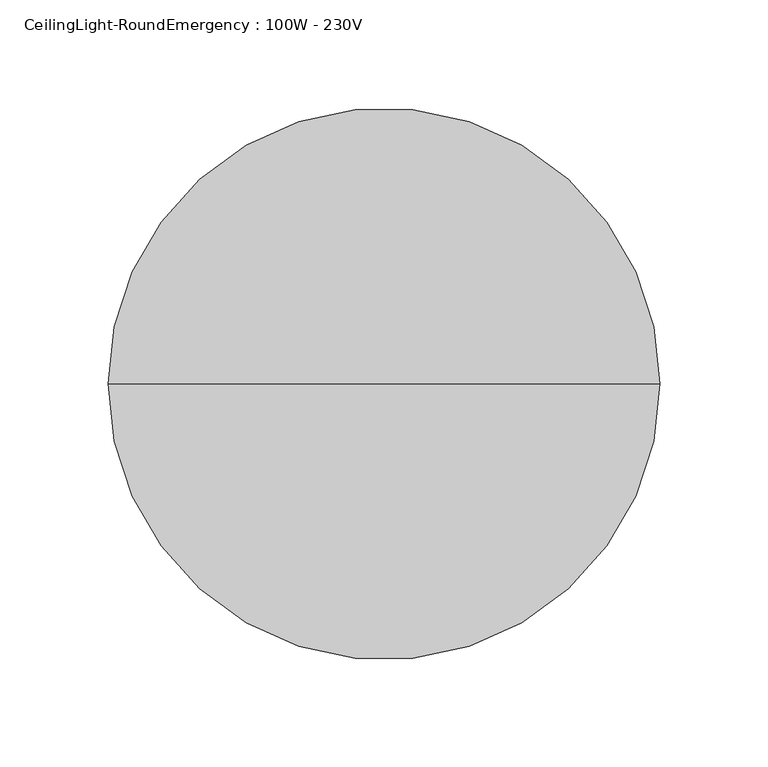
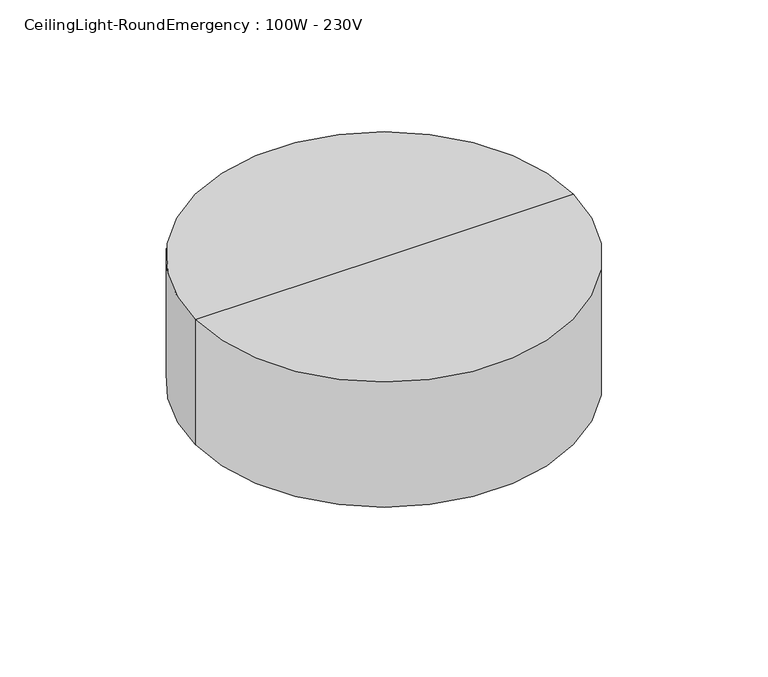
"""IFC4 building model written with IfcOpenShell, lengths in millimetres: light fixture geometry, CeilingLight-RoundEmergency : 100W - 230V."""

from ifc_helpers import new_model, si_unit, point, frame, origin, origin_2d, place, context, project, spatial, polyline, circle_curve, trimmed, segment, composite_curve, outline, extrude, source, transform, mapped, element, save
from ifc_brep_helpers import plane_surface, cylinder_surface, revolved_surface, advanced_brep


def ceilinglight_roundemergency_100w_230v_36b39b3f(model_context):
    return source(origin(), model_context, "Body", "SolidModel", [
        extrude(outline(composite_curve([segment(trimmed(circle_curve(origin_2d(), 82.55), [point((-82.55, 0.0))], [point((82.55, 0.0))], False, "CARTESIAN"), True, "CONTINUOUS"), segment(trimmed(circle_curve(origin_2d(), 82.55), [point((82.55, 0.0))], [point((-82.55, 0.0))], False, "CARTESIAN"), True, "CONTINUOUS")], self_intersect=False), holes=[composite_curve([segment(trimmed(circle_curve(origin_2d(), 76.2), [point((-76.2, 0.0))], [point((76.2, 0.0))], True, "CARTESIAN"), True, "CONTINUOUS"), segment(trimmed(circle_curve(origin_2d(), 76.2), [point((76.2, 0.0))], [point((-76.2, 0.0))], True, "CARTESIAN"), True, "CONTINUOUS")], self_intersect=False)]), frame((0.0, 0.0, -101.810254), z_axis=(0.0, 0.0, 1.0), x_axis=(1.0, 0.0, 0.0)), (0.0, 0.0, 1.0), 25.0),
        advanced_brep(
        [(127.0, 0.0, -74.6), (-127.0, 0.0, -74.6), (-127.0, 0.0, 14.3), (127.0, 0.0, 14.3), (76.2, 0.0, -74.6), (-76.2, 0.0, -74.6), (76.2, 0.0, -100.0), (-76.2, 0.0, -100.0), (73.025, 0.0, -100.0), (-73.025, 0.0, -100.0), (73.025, 0.0, -71.425), (-73.025, 0.0, -71.425), (123.825, 0.0, -71.425), (-123.825, 0.0, -71.425), (123.825, 0.0, 11.125), (-123.825, 0.0, 11.125), (0.0, 0.0, 11.125), (0.0, 0.0, 14.3)],
        [
            (0, 1, circle_curve(frame((0.0, 0.0, -74.6), z_axis=(0.0, 0.0, 1.0), x_axis=(-1.0, 0.0, 0.0)), 127.0)),
            (1, 2),
            (2, 3, circle_curve(frame((0.0, 0.0, 14.3), z_axis=(0.0, 0.0, -1.0), x_axis=(-1.0, 0.0, 0.0)), 127.0)),
            (3, 0),
            (1, 0, circle_curve(frame((0.0, 0.0, -74.6), z_axis=(0.0, 0.0, 1.0), x_axis=(-1.0, 0.0, 0.0)), 127.0)),
            (3, 2, circle_curve(frame((0.0, 0.0, 14.3), z_axis=(0.0, 0.0, -1.0), x_axis=(-1.0, 0.0, 0.0)), 127.0)),
            (4, 5, circle_curve(frame((0.0, 0.0, -74.6), z_axis=(0.0, 0.0, 1.0), x_axis=(-1.0, 0.0, 0.0)), 76.2)),
            (5, 1),
            (0, 4),
            (5, 4, circle_curve(frame((0.0, 0.0, -74.6), z_axis=(0.0, 0.0, 1.0), x_axis=(-1.0, 0.0, 0.0)), 76.2)),
            (6, 7, circle_curve(frame((0.0, 0.0, -100.0), z_axis=(0.0, 0.0, 1.0), x_axis=(-1.0, 0.0, 0.0)), 76.2)),
            (7, 5),
            (4, 6),
            (7, 6, circle_curve(frame((0.0, 0.0, -100.0), z_axis=(0.0, 0.0, 1.0), x_axis=(-1.0, 0.0, 0.0)), 76.2)),
            (8, 9, circle_curve(frame((0.0, 0.0, -100.0), z_axis=(0.0, 0.0, 1.0), x_axis=(-1.0, 0.0, 0.0)), 73.025)),
            (9, 7),
            (6, 8),
            (9, 8, circle_curve(frame((0.0, 0.0, -100.0), z_axis=(0.0, 0.0, 1.0), x_axis=(-1.0, 0.0, 0.0)), 73.025)),
            (10, 11, circle_curve(frame((0.0, 0.0, -71.425), z_axis=(0.0, 0.0, 1.0), x_axis=(-1.0, 0.0, 0.0)), 73.025)),
            (11, 9),
            (8, 10),
            (11, 10, circle_curve(frame((0.0, 0.0, -71.425), z_axis=(0.0, 0.0, 1.0), x_axis=(-1.0, 0.0, 0.0)), 73.025)),
            (12, 13, circle_curve(frame((0.0, 0.0, -71.425), z_axis=(0.0, 0.0, 1.0), x_axis=(-1.0, 0.0, 0.0)), 123.825)),
            (13, 11),
            (10, 12),
            (13, 12, circle_curve(frame((0.0, 0.0, -71.425), z_axis=(0.0, 0.0, 1.0), x_axis=(-1.0, 0.0, 0.0)), 123.825)),
            (14, 15, circle_curve(frame((0.0, 0.0, 11.125), z_axis=(0.0, 0.0, 1.0), x_axis=(-1.0, 0.0, 0.0)), 123.825)),
            (15, 13),
            (12, 14),
            (15, 14, circle_curve(frame((0.0, 0.0, 11.125), z_axis=(0.0, 0.0, 1.0), x_axis=(-1.0, 0.0, 0.0)), 123.825)),
            (16, 15),
            (14, 16),
            (2, 17),
            (17, 3),
        ],
        [
            cylinder_surface(frame((0.0, 0.0, 11.125), z_axis=(0.0, 0.0, -1.0), x_axis=(-1.0, 0.0, 0.0)), 127.0),
            plane_surface(frame((0.0, 0.0, -74.6), z_axis=(0.0, 0.0, -1.0), x_axis=(-1.0, 0.0, 0.0))),
            cylinder_surface(frame((0.0, 0.0, 11.125), z_axis=(0.0, 0.0, -1.0), x_axis=(-1.0, 0.0, 0.0)), 76.2),
            plane_surface(frame((0.0, 0.0, -100.0), z_axis=(0.0, 0.0, -1.0), x_axis=(-1.0, 0.0, 0.0))),
            revolved_surface(polyline([(-73.025, 0.0, -100.0), (-73.025, 0.0, -71.425)]), (0.0, 0.0, 11.125), (0.0, 0.0, -1.0)),
            plane_surface(frame((0.0, 0.0, -71.425), z_axis=(0.0, 0.0, 1.0), x_axis=(-1.0, 0.0, 0.0))),
            revolved_surface(polyline([(-123.825, 0.0, -71.425), (-123.825, 0.0, 11.125)]), (0.0, 0.0, 11.125), (0.0, 0.0, -1.0)),
            plane_surface(frame((0.0, 0.0, 11.125), z_axis=(0.0, 0.0, -1.0), x_axis=(-1.0, 0.0, 0.0))),
            plane_surface(frame((0.0, 0.0, 14.3), z_axis=(0.0, 0.0, 1.0), x_axis=(-1.0, 0.0, 0.0))),
        ],
        [
            (0, [[1, 2, 3, 4]]),
            (0, [[5, -4, 6, -2]]),
            (1, [[7, 8, -1, 9]]),
            (1, [[10, -9, -5, -8]]),
            (2, [[11, 12, -7, 13]]),
            (2, [[14, -13, -10, -12]]),
            (3, [[15, 16, -11, 17]]),
            (3, [[18, -17, -14, -16]]),
            (4, [[19, 20, -15, 21]]),
            (4, [[22, -21, -18, -20]]),
            (5, [[23, 24, -19, 25]]),
            (5, [[26, -25, -22, -24]]),
            (6, [[27, 28, -23, 29]]),
            (6, [[30, -29, -26, -28]]),
            (7, [[31, -27, 32]]),
            (7, [[-32, -30, -31]]),
            (8, [[-3, 33, 34]]),
            (8, [[-6, -34, -33]]),
        ],
    ),
    ])


if __name__ == "__main__":
    model = new_model("IFC4")
    model_context = context("Model", 3, world=origin())
    ifc_project = project(units=[si_unit("LENGTHUNIT", "METRE", prefix="MILLI")], contexts=[model_context])
    site = spatial("IfcSite", under=ifc_project)
    building = spatial("IfcBuilding", under=site)
    placement = place(None, origin())
    ceilinglight_roundemergency_100w_230v_shape = ceilinglight_roundemergency_100w_230v_36b39b3f(model_context)
    element("IfcLightFixture", 1, ObjectType="CeilingLight-RoundEmergency : 100W - 230V", at=placement, inside=building, context=model_context, shape_type="MappedRepresentation", body=[
        mapped(ceilinglight_roundemergency_100w_230v_shape, transform((0.0, 0.0, 0.0), x_axis=(1.0, 0.0, 0.0), y_axis=(0.0, 1.0, 0.0), z_axis=(0.0, 0.0, 1.0))),
    ])
    save(model, "model.ifc")

# Revit data of these elements
# Type "CeilingLight-RoundEmergency : 100W - 230V"
#   Type Mark = "CeilingLight-RoundEmergencyB"
#   Classification.OmniClass.21.Number = "21-04 50 40 50"
#   Classification.OmniClass.21.Description = "Lighting Fixtures"
#   Classification.UniFormat.II.Description = "Lighting Fixtures"
#   Classification.OmniClass.23.Number = "23-35 47 13"
#   Classification.OmniClass.23.Description = "Emergency Lighting"
#   Classification.UniFormat.II.Number = "D5040.50"
#   COBie.Type.CreatedBy = "info@mma.ie"
#   COBie.Type.CreatedOn = "2017-07-25T10:15:16"
#   COBie.Type.Name = "CeilingLight-RoundEmergencyB"
#   COBie.Type.Category = "23-35 47 13 : Emergency Lighting"
#   COBie.Type.Description = "CeilingLight-RoundEmergency_100W - 230V"
#   COBie.Type.AssetType = "Fixed"
#   COBie.Type.Manufacturer = ""
#   COBie.Type.ModelNumber = ""
#   Keynote = "26 52 00.B"
#   Lamp = "A-19"
#   Photometric Web File = "CLFR1A21.ies"
#   Assembly Code = "D5020220"
#   COBie.Type.ReplacementCost = 0
#   Wattage = 100 W
#   built-in parameter 1150110 = 1 (stored number, unit not read)
#   built-in parameter 1150109 = 1 (stored number, unit not read)
#   built-in parameter 1150113 = 1 (stored number, unit not read)
#   Tilt Angle = -90.00°
#   built-in parameter 1150115 = 1 (stored number, unit not read)
#   built-in parameter 1150105 = 139.261 (stored number, unit not read)
#   built-in parameter 1150112 = 1 (stored number, unit not read)
#   built-in parameter 1150114 = 1 (stored number, unit not read)
#   built-in parameter 1150107 = 2800 (stored number, unit not read)
#   built-in parameter 1150106 = 1.39261 (stored number, unit not read)
#   Emit from Circle Diameter = 254 mm
#   built-in parameter 1150104 = 1.6258 (stored number, unit not read)
#   E.C.L. Efficacy = 17.5 lm/W
#   E.C.L. Diameter = 254 mm
#   Lumens = 1750 lm
#   built-in parameter 1114217 = 1 (stored number, unit not read)
#   Default Elevation = 1200 mm
#   Ballast Voltage = 230 V
#   built-in parameter 1114218 = 1 (stored number, unit not read)
#   built-in parameter 1150133 = 10 (stored number, unit not read)
#   Apparent Load = 100 VA
#   COBie.Type = yes
#   built-in parameter 1150134 = 4
#   built-in parameter 1150137 = 1
#   Color Filter = 16777215
#   built-in parameter 1140040 [instance default] = 1
#   Ballast Number of Poles = 1
#   black = Glass - White, High Luminance
#   Load Classification = Lighting - Dwelling Unit
#   Light Box Material = Metal - Paint Finish - Dark Grey, Matt
#   E.C.L. Material = Metal - Paint Finish - Dark Grey, Matt
#   Diffuser Material = Glass - White, High Luminance
#   Emit Shape Visible in Rendering = no
#   Dimming Lamp Color Temperature Shift = (empty or 0)
# Element 1 (IfcLightFixture, "CeilingLight-RoundEmergency : 100W - 230V")
#   Materials on its faces: "Glass - White, High Luminance", "Metal - Paint Finish - Dark Grey, Matt"
# Materials
#   "Glass - White, High Luminance": class "Glass", colour RGB 249 250 249, transparency 0.8
#   "Metal - Paint Finish - Dark Grey, Matt": class "Paint", colour RGB 98 98 98, transparency 0
